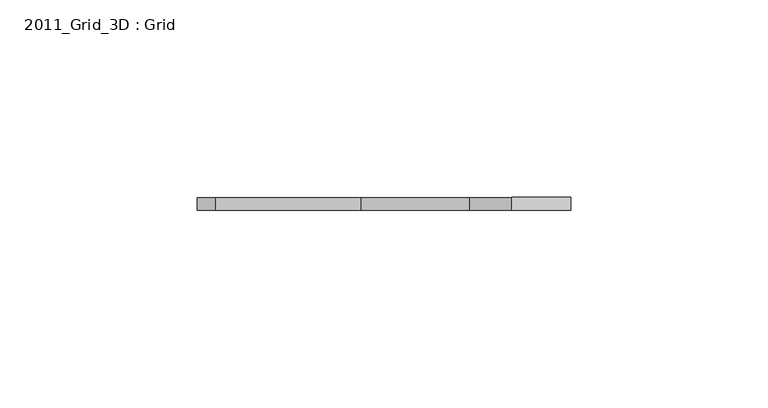
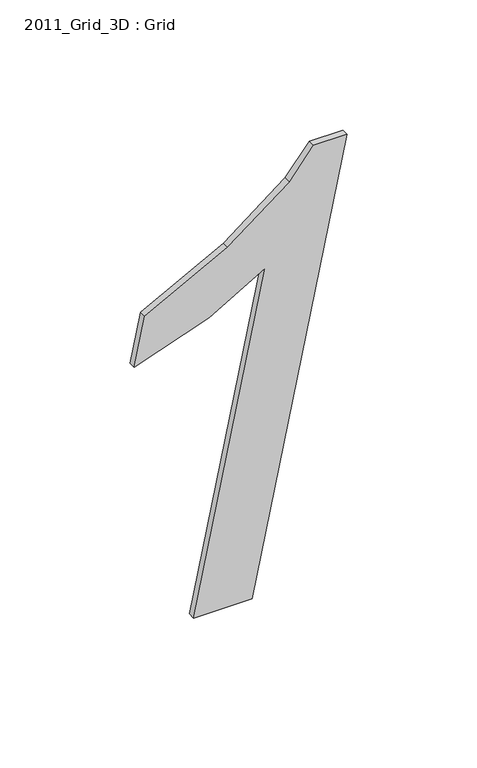
"""IFC4 building model written with IfcOpenShell, lengths in millimetres: proxy geometry, 2011_Grid_3D : Grid."""

from ifc_helpers import new_model, si_unit, frame, origin, place, context, project, spatial, polyline, outline, extrude, source, transform, mapped, element, save


def proxy_2011_grid_3d_grid_8daef3c7(model_context):
    return source(origin(), model_context, "Body", "SweptSolid", [
        extrude(outline(polyline([(-101.6, 32359.573927), (-101.6, 32385.4006614), (101.4447294, 32427.5859799), (101.4447294, 32412.7641112), (88.0108618, 32402.0071029), (67.0173455, 32374.5692958), (47.5109731, 32337.8120529), (25.3029559, 32333.152335), (36.729179, 32366.4271823), (51.3775476, 32391.299666), (-101.6, 32359.573927)])), frame((0.0, -3.175, 0.0), z_axis=(0.0, 1.0, 0.0), x_axis=(0.0, 0.0, 1.0)), (0.0, 0.0, 1.0), 3.175),
    ])


if __name__ == "__main__":
    model = new_model("IFC4")
    model_context = context("Model", 3, world=origin())
    ifc_project = project(units=[si_unit("LENGTHUNIT", "METRE", prefix="MILLI")], contexts=[model_context])
    site = spatial("IfcSite", under=ifc_project)
    building = spatial("IfcBuilding", under=site)
    placement = place(None, origin())
    proxy_2011_grid_3d_grid_shape = proxy_2011_grid_3d_grid_8daef3c7(model_context)
    element("IfcBuildingElementProxy", 1, Name="2011_Grid_3D : Grid", ObjectType="2011_Grid_3D : Grid", at=placement, inside=building, context=model_context, shape_type="MappedRepresentation", body=[
        mapped(proxy_2011_grid_3d_grid_shape, transform((0.0, 0.0, 0.0), x_axis=(1.0, 0.0, 0.0), y_axis=(0.0, 1.0, 0.0), z_axis=(0.0, 0.0, 1.0))),
    ])
    save(model, "model.ifc")

# Revit data of these elements
# Type "2011_Grid_3D : Grid"
#   Workplane [instance default] = "LEVEL"
#   Grid [instance default] = "S"
#   t [instance default] = 12' - 6"
#   built-in parameter 1001306 [instance default] = 50 (stored number, unit not read)
#   d [instance default] = 2
#   Symbol At End 2 [instance default] = yes
#   Symbol At End 1 [instance default] = yes
#   Robust [instance default] = yes
#   No of grid markers [instance default] = 3
#   Grid Height Visible = yes
#   Height = 0
#   Assembly Code = ""
# Element 1 (IfcBuildingElementProxy, "2011_Grid_3D : Grid")
#   Workplane = "1"
#   Grid = "1"
#   t = 13' - 2.15638"
#   built-in parameter 1001306 = 105.438 (stored number, unit not read)
#   d = 4
#   Robust = no
#   No of grid markers = 5
#   Materials on its faces: "Letter"
# Materials
#   "Letter": class "Unassigned", colour RGB 178 187 30, transparency 0, Comments = "Rendering appearance not upgraded "
